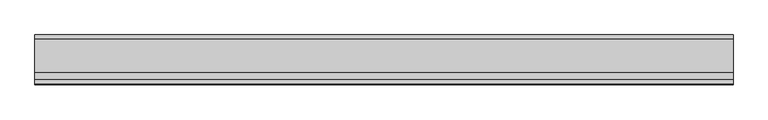
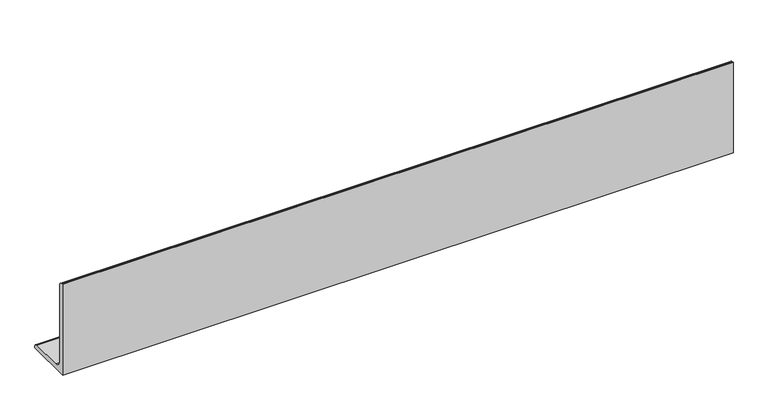
"""IFC4 building model written with IfcOpenShell, lengths in millimetres: beam geometry, NLRS_28_SF_LIB_stalen ligger hoekprofiel ongelijkzijdig-AV-MMBS-SRP_gen_rsf : stalen ligger ongelijzijdig hoekprofiel LUEQ_gen__200x100x10."""

from ifc_helpers import new_model, si_unit, point, frame, frame_2d, origin, place, context, project, spatial, polyline, circle_curve, trimmed, segment, composite_curve, outline, extrude, source, transform, mapped, element, save


def beam_09181c89(model_context):
    return source(origin(), model_context, "Body", "SweptSolid", [
        extrude(outline(composite_curve([segment(polyline([(-20.13, -69.3), (-20.13, 130.7), (-17.63, 130.7)]), True, "CONTINUOUS"), segment(trimmed(circle_curve(frame_2d((-17.63, 123.2)), 7.5), [point((-17.63, 130.7))], [point((-10.13, 123.2))], False, "CARTESIAN"), True, "CONTINUOUS"), segment(polyline([(-10.13, 123.2), (-10.13, -44.3)]), True, "CONTINUOUS"), segment(trimmed(circle_curve(frame_2d((4.87, -44.3)), 15.0), [point((-10.13, -44.3))], [point((4.87, -59.3))], True, "CARTESIAN"), True, "CONTINUOUS"), segment(polyline([(4.87, -59.3), (72.37, -59.3)]), True, "CONTINUOUS"), segment(trimmed(circle_curve(frame_2d((72.37, -66.8)), 7.5), [point((72.37, -59.3))], [point((79.87, -66.8))], False, "CARTESIAN"), True, "CONTINUOUS"), segment(polyline([(79.87, -66.8), (79.87, -69.3), (-20.13, -69.3)]), True, "CONTINUOUS")], self_intersect=False)), frame((-700.0, 0.0, 0.0), z_axis=(1.0, 0.0, 0.0), x_axis=(0.0, 1.0, 0.0)), (0.0, 0.0, 1.0), 1400.0),
    ])


if __name__ == "__main__":
    model = new_model("IFC4")
    model_context = context("Model", 3, world=origin())
    ifc_project = project(units=[si_unit("LENGTHUNIT", "METRE", prefix="MILLI")], contexts=[model_context])
    site = spatial("IfcSite", under=ifc_project)
    building = spatial("IfcBuilding", under=site)
    placement = place(None, origin())
    beam_shape = beam_09181c89(model_context)
    element("IfcBeam", 1, ObjectType="NLRS_28_SF_LIB_stalen ligger hoekprofiel ongelijkzijdig-AV-MMBS-SRP_gen_rsf : stalen ligger ongelijzijdig hoekprofiel LUEQ_gen__200x100x10", at=placement, inside=building, context=model_context, shape_type="MappedRepresentation", body=[
        mapped(beam_shape, transform((0.0, 0.0, 0.0), x_axis=(1.0, 0.0, 0.0), y_axis=(0.0, 1.0, 0.0), z_axis=(0.0, 0.0, 1.0))),
    ])
    save(model, "model.ifc")

# Revit data of these elements
# Type "NLRS_28_SF_LIB_stalen ligger hoekprofiel ongelijkzijdig-AV-MMBS-SRP_gen_rsf : stalen ligger ongelijzijdig hoekprofiel LUEQ_gen__200x100x10"
#   Type IfcGUID = "0dxhH9VHH5jh7XQ0uLfXuR"
#   IfcExportAs = "IfcBeamType"
#   Type Comments = "L200x100x10"
#   Model = " "
#   Manufacturer = " "
#   Fire Rating = " "
#   Description = "stalen ligger L200x100x10"
#   Assembly Code = "28.11"
#   vz = 130.7 mm
#   vy = 79.87 mm
#   tw = 10 mm
#   tf = 10 mm
#   ri = 7.5 mm
#   ra = 15 mm
#   d = 200 mm
#   bf = 100 mm
#   NLRS_C_lengte [instance default] = 1524 mm
#   Length [instance default] = 1524 mm
#   Structural Material = NLRS_h2_staal_gen_rsf
#   Keynote = ""
# Element 1 (IfcBeam, "NLRS_28_SF_LIB_stalen ligger hoekprofiel ongelijkzijdig-AV-MMBS-SRP_gen_rsf : stalen ligger ongelijzijdig hoekprofiel LUEQ_gen__200x100x10")
#   NLRS_C_lengte = 1400 mm
#   Materials on its faces: "NLRS_h2_staal_gen_rsf"
# Materials
#   "NLRS_h2_staal_gen_rsf": class "H - Metaal", colour RGB 189 187 185, transparency 0, Keynote = "h2", Manufacturer = "Revit Standards Foundation", URL = "www.revitstandards.org", Description = "staal", Cost = 0
